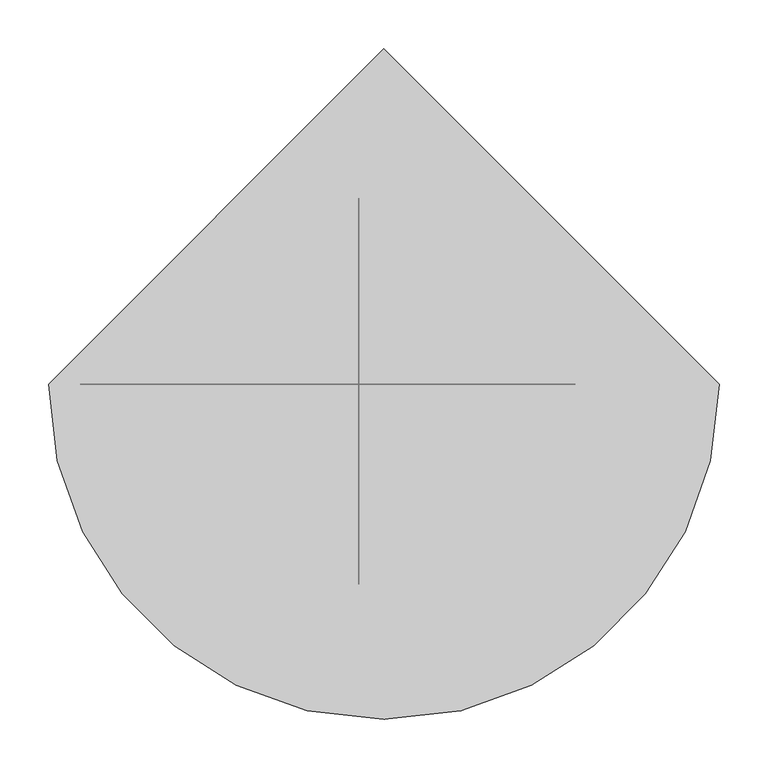
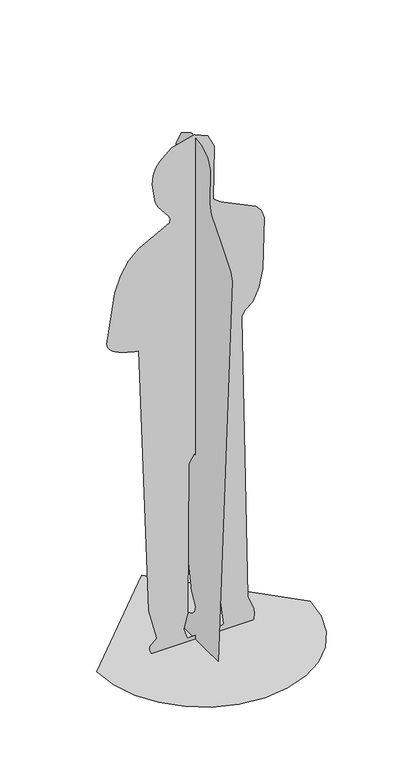
"""IFC4 building model written with IfcOpenShell, lengths in millimetres: proxy geometry, jay 23630 : jay 23630."""

from ifc_helpers import new_model, si_unit, origin, place, context, project, spatial, triangles, source, transform, mapped, element, save


def entourage_8fcae429(model_context):
    return source(origin(), model_context, "Body", "Tessellation", [
        triangles([(-345.573129, 0.0, 0.0), (-336.4372767, -79.1825214, 0.0), (-310.4185887, -151.898995, 0.0), (-269.6002954, -216.0660267, 0.0), (-216.0660449, -269.6003499, 0.0), (-151.8989496, -310.4185161, 0.0), (-79.182476, -336.4372767, 0.0), (1.51e-05, -345.573129, 0.0), (79.1825214, -336.4373131, 0.0), (151.8990041, -310.4185887, 0.0), (216.0660449, -269.6002954, 0.0), (269.6004044, -216.0660449, 0.0), (310.4185524, -151.8989405, 0.0), (336.4372767, -79.1824669, 0.0), (345.573129, 3.02e-05, 0.0), (-4.53e-05, 345.573129, 0.0), (-25.78036, -206.1897945, 1348.8136002), (-25.78036, -197.5853052, 1374.9567719), (-25.78036, -143.9297776, 1440.4177471), (-25.78036, -88.0519655, 1504.3160271), (-25.78036, -79.0557305, 1537.7600613), (-25.78036, -83.3728362, 1655.4464825), (-25.78036, -70.0856975, 1687.5603653), (-25.78036, -36.8546772, 1709.6662834), (-25.78036, 23.8686285, 1717.8949963), (-25.78036, 79.9018998, 1684.0287495), (-25.78036, 106.2359483, 1634.1418236), (-25.78036, 109.3285375, 1576.3372124), (-25.78036, 95.6374309, 1518.7173283), (-25.78036, 71.6204603, 1469.3858917), (-25.78036, 43.7353573, 1436.4453152), (-25.78036, 18.439931, 1427.9987377), (-25.78036, 12.9047356, 1418.4000504), (-25.78036, 17.9030394, 1403.9002087), (-25.78036, 100.3158972, 1305.1847225), (-25.78036, 139.8422273, 1319.3011574), (-25.78036, 147.3154902, 1313.5241844), (-25.78036, 153.4761334, 1298.3650806), (-25.78036, 159.5450399, 1229.1756992), (-25.78036, 155.917754, 1209.0686417), (-25.78036, 148.709137, 1195.8695927), (-25.78036, 191.504717, 912.7641987), (-25.78036, 185.9813623, 822.2158739), (-25.78036, 168.0753332, 726.406097), (-25.78036, 163.1484355, 723.9989765), (-25.78036, 157.8330986, 724.045776), (-25.78036, 131.3723318, 737.6993757), (-25.78036, 21.417554, 149.8941936), (-25.78036, -1.3232615, 110.9245429), (-25.78036, 4.0590798, 90.9092221), (-25.78036, 18.2062061, 77.7815168), (-25.78036, 83.2378244, 46.7363279), (-25.78036, 102.4456182, 28.1713909), (-25.78036, 115.4189542, 0.0001939), (-25.78036, -127.8900044, 0.0001939), (-47.6681978, 5.01e-05, 607.394684), (-50.5685249, 7.96e-05, 98.4130518), (-63.1404637, 8.25e-05, 45.9886491), (-51.8472214, 8.45e-05, 12.1089164), (63.743988, 8.33e-05, 17.5652887), (66.5308818, 8.31e-05, 21.3655518), (-8.2278249, 5.05e-05, 609.0638409), (-29.2607276, 4.73e-05, 636.0603762), (-172.7832943, 8.44e-05, 13.4467537), (-173.6616201, 8.39e-05, 22.9478476), (-170.9381671, 8.35e-05, 29.5787746), (-154.6519156, 8.27e-05, 42.9999871), (-151.0159457, 8.23e-05, 48.9000085), (-176.6022473, 7.63e-05, 150.451091), (-208.3969635, 2.09e-05, 1050.4165524), (-216.4831887, 2.08e-05, 1051.9022175), (-226.3935031, 2.06e-05, 1053.8479563), (-237.6114049, 2.05e-05, 1056.3359585), (-249.6203194, 2.03e-05, 1059.4489225), (-261.9037993, 2.01e-05, 1063.2688929), (-273.9452518, 1.99e-05, 1067.8781319), (-285.228175, 1.97e-05, 1073.35912), (-292.7744804, 1.95e-05, 1078.0168299), (-299.4163715, 1.93e-05, 1083.228503), (-304.945558, 1.92e-05, 1089.0273497), (-309.1536223, 1.9e-05, 1095.4465799), (-311.8324196, 1.88e-05, 1102.5192587), (-312.7733505, 1.87e-05, 1110.2786688), (-311.7682157, 1.85e-05, 1118.7580204), (-286.8266966, 1.73e-05, 1275.1930939), (-267.1756069, 1.34e-05, 1328.1942192), (-240.945322, 8.5e-06, 1369.0343136), (-206.7917381, 3.8e-06, 1401.2005188), (-109.3374395, -1e-06, 1453.4599743), (-107.2218801, -2e-06, 1465.6289989), (-111.9356912, -3.4e-06, 1476.9063629), (-145.5691942, -7.6e-06, 1518.8280773), (-156.1162521, -8.3e-06, 1539.9788212), (-165.8142066, -1.06e-05, 1603.881752), (-162.2941272, -1.25e-05, 1633.2779228), (-153.7863434, -1.38e-05, 1656.3025349), (-141.886879, -1.48e-05, 1674.1116222), (-101.7987827, -1.66e-05, 1707.8037518), (-29.8635274, -1.51e-05, 1727.1999516), (13.7644623, -1.3e-05, 1708.5696934), (35.5195707, -1.05e-05, 1664.4861923), (32.4991723, -3.3e-06, 1485.0823174), (52.4866355, -2.3e-06, 1467.9128712), (169.1693616, 1.1e-06, 1411.612674), (187.957677, 2.2e-06, 1392.5309898), (197.4322985, 4e-06, 1363.4756413), (192.0197292, 1.43e-05, 1189.9500412), (178.7207045, 1.78e-05, 1132.0744314), (159.5661324, 2.03e-05, 1088.5580469), (134.4912548, 2.16e-05, 1068.0268147), (124.9300924, 2.55e-05, 1049.9808231), (143.8918166, 8.04e-05, 86.7553968), (162.7830327, 8.38e-05, 38.1705126), (165.3513534, 8.45e-05, 22.7356648), (163.2783513, 8.52e-05, 0.0004369), (-166.9538173, 8.52e-05, 0.0004369)], [[15, 16, 1], [14, 15, 1], [14, 1, 2], [13, 14, 2], [13, 2, 3], [13, 3, 4], [12, 13, 4], [11, 12, 4], [11, 4, 5], [11, 5, 6], [11, 6, 7], [11, 7, 8], [11, 8, 9], [11, 9, 10], [53, 54, 55], [52, 53, 55], [51, 52, 55], [50, 51, 55], [49, 50, 55], [48, 49, 55], [47, 48, 55], [47, 55, 17], [35, 36, 37], [35, 37, 38], [35, 38, 39], [43, 44, 45], [43, 45, 46], [43, 46, 47], [43, 47, 17], [42, 43, 17], [41, 42, 17], [41, 17, 18], [41, 18, 19], [40, 41, 19], [39, 40, 19], [35, 39, 19], [34, 35, 19], [33, 34, 19], [33, 19, 20], [32, 33, 20], [32, 20, 21], [31, 32, 21], [30, 31, 21], [29, 30, 21], [28, 29, 21], [27, 28, 21], [26, 27, 21], [25, 26, 21], [24, 25, 21], [24, 21, 22], [23, 24, 22], [114, 115, 116], [57, 58, 68], [57, 68, 69], [56, 57, 69], [56, 69, 70], [63, 56, 70], [68, 58, 59], [67, 68, 59], [66, 67, 59], [65, 66, 59], [64, 65, 59], [116, 64, 59], [99, 100, 101], [98, 99, 101], [97, 98, 101], [96, 97, 101], [95, 96, 101], [94, 95, 101], [93, 94, 101], [92, 93, 101], [91, 92, 101], [91, 101, 102], [90, 91, 102], [89, 90, 102], [89, 102, 103], [108, 109, 110], [104, 105, 106], [103, 104, 106], [89, 103, 106], [89, 106, 107], [89, 107, 108], [89, 108, 110], [88, 89, 110], [87, 88, 110], [86, 87, 110], [85, 86, 110], [84, 85, 110], [84, 110, 111], [83, 84, 111], [82, 83, 111], [81, 82, 111], [80, 81, 111], [79, 80, 111], [78, 79, 111], [77, 78, 111], [76, 77, 111], [75, 76, 111], [74, 75, 111], [73, 74, 111], [72, 73, 111], [71, 72, 111], [70, 71, 111], [63, 70, 111], [62, 63, 111], [61, 62, 111], [61, 111, 112], [61, 112, 113], [61, 113, 114], [60, 61, 114], [60, 114, 116], [60, 116, 59]], closed=False),
    ])


if __name__ == "__main__":
    model = new_model("IFC4")
    model_context = context("Model", 3, world=origin())
    ifc_project = project(units=[si_unit("LENGTHUNIT", "METRE", prefix="MILLI")], contexts=[model_context])
    site = spatial("IfcSite", under=ifc_project)
    building = spatial("IfcBuilding", under=site)
    placement = place(None, origin())
    entourage_shape = entourage_8fcae429(model_context)
    element("IfcBuildingElementProxy", 1, Name="jay 23630 : jay 23630", ObjectType="jay 23630 : jay 23630", at=placement, inside=building, context=model_context, shape_type="MappedRepresentation", body=[
        mapped(entourage_shape, transform((0.0, 0.0, 0.0), x_axis=(1.0, 0.0, 0.0), y_axis=(0.0, 1.0, 0.0), z_axis=(0.0, 0.0, 1.0))),
    ])
    save(model, "model.ifc")

# Revit data of these elements
# Type "jay 23630 : jay 23630"
#   built-in parameter 1005195 = "RPC-8-FWF3-6VPX-GP75-J"
#   Height = 0
